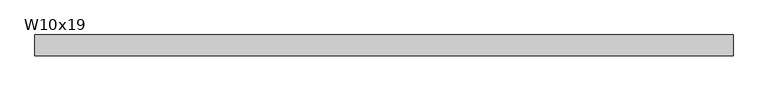
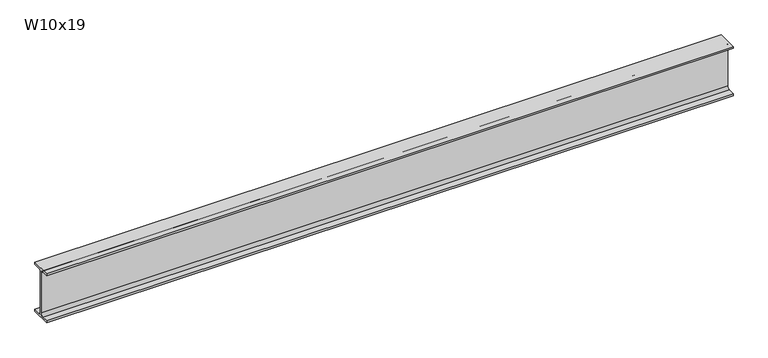
"""IFC4 building model written with IfcOpenShell, lengths in millimetres: beam geometry, RME W-Wide Flange : W10x19."""

from ifc_helpers import new_model, si_unit, point, frame, frame_2d, origin, place, context, project, spatial, polyline, circle_curve, trimmed, segment, composite_curve, outline, extrude, source, transform, mapped, element, save


def w10x19_840bb0a0(model_context):
    return source(origin(), model_context, "Body", "SweptSolid", [
        extrude(outline(composite_curve([segment(polyline([(51.054, -119.507), (51.054, -129.54), (-51.054, -129.54), (-51.054, -119.507), (-16.9545, -119.507)]), True, "CONTINUOUS"), segment(trimmed(circle_curve(frame_2d((-16.9545, -105.7275)), 13.7795), [point((-16.9545, -119.507))], [point((-3.175, -105.7275))], True, "CARTESIAN"), True, "CONTINUOUS"), segment(polyline([(-3.175, -105.7275), (-3.175, 105.7275)]), True, "CONTINUOUS"), segment(trimmed(circle_curve(frame_2d((-16.9545, 105.7275)), 13.7795), [point((-3.175, 105.7275))], [point((-16.9545, 119.507))], True, "CARTESIAN"), True, "CONTINUOUS"), segment(polyline([(-16.9545, 119.507), (-51.054, 119.507), (-51.054, 129.54), (51.054, 129.54), (51.054, 119.507), (16.9545, 119.507)]), True, "CONTINUOUS"), segment(trimmed(circle_curve(frame_2d((16.9545, 105.7275)), 13.7795), [point((16.9545, 119.507))], [point((3.175, 105.7275))], True, "CARTESIAN"), True, "CONTINUOUS"), segment(polyline([(3.175, 105.7275), (3.175, -105.7275)]), True, "CONTINUOUS"), segment(trimmed(circle_curve(frame_2d((16.9545, -105.7275)), 13.7795), [point((3.175, -105.7275))], [point((16.9545, -119.507))], True, "CARTESIAN"), True, "CONTINUOUS"), segment(polyline([(16.9545, -119.507), (51.054, -119.507)]), True, "CONTINUOUS")], self_intersect=False)), frame((-1736.5321927, 0.0, 0.0), z_axis=(1.0, 0.0, 0.0), x_axis=(0.0, 1.0, 0.0)), (0.0, 0.0, 1.0), 3438.9182322),
    ])


if __name__ == "__main__":
    model = new_model("IFC4")
    model_context = context("Model", 3, world=origin())
    ifc_project = project(units=[si_unit("LENGTHUNIT", "METRE", prefix="MILLI")], contexts=[model_context])
    site = spatial("IfcSite", under=ifc_project)
    building = spatial("IfcBuilding", under=site)
    placement = place(None, origin())
    w10x19_shape = w10x19_840bb0a0(model_context)
    element("IfcBeam", 1, ObjectType="RME W-Wide Flange : W10x19", at=placement, inside=building, context=model_context, shape_type="MappedRepresentation", body=[
        mapped(w10x19_shape, transform((0.0, 0.0, 0.0), x_axis=(1.0, 0.0, 0.0), y_axis=(0.0, 1.0, 0.0), z_axis=(0.0, 0.0, 1.0))),
    ])
    save(model, "model.ifc")

# Revit data of these elements
# Type "RME W-Wide Flange : W10x19"
#   WELD P [instance default] = ""
#   WELD LE [instance default] = ""
#   WELD D [instance default] = ""
#   TOP SECTION SIZE [instance default] = ""
#   TOP SECTION LENGTH [instance default] = ""
#   REMARKS [instance default] = ""
#   REINF TYPE [instance default] = ""
#   Nominal Size = "W24"
#   End Bearing Capacity [instance default] = ""
#   BOT SECTION SIZE [instance default] = ""
#   BOT SECTION LENGTH [instance default] = ""
#   Assembly Code = "B10"
#   W = 19
#   Start Extension Calculation [instance default] = 10' - 0"
#   Start Extension [instance default] = -0' - 0 1/2"
#   End Extension Calculation [instance default] = 10' - 0"
#   End Extension [instance default] = -0' - 0 1/2"
#   Length [instance default] = 5' - 0"
#   bf = 0' - 4.02"
#   d = 0' - 10.2"
#   k = 0' - 0 15/16"
#   k2 = 0' - 0.5425"
#   tf = 0' - 0.395"
#   tw = 0' - 0 1/4"
#   A = 0.0390278 SF
#   Structural Material [instance default] = Metal - Steel - ASTM A992
# Element 1 (IfcBeam, "RME W-Wide Flange : W10x19")
#   Length = 11' - 10.55345"
#   Materials on its faces: "Metal - Steel - ASTM A992"
# Materials
#   "Metal - Steel - ASTM A992": class "Metal", colour RGB 255 128 0, transparency 0
